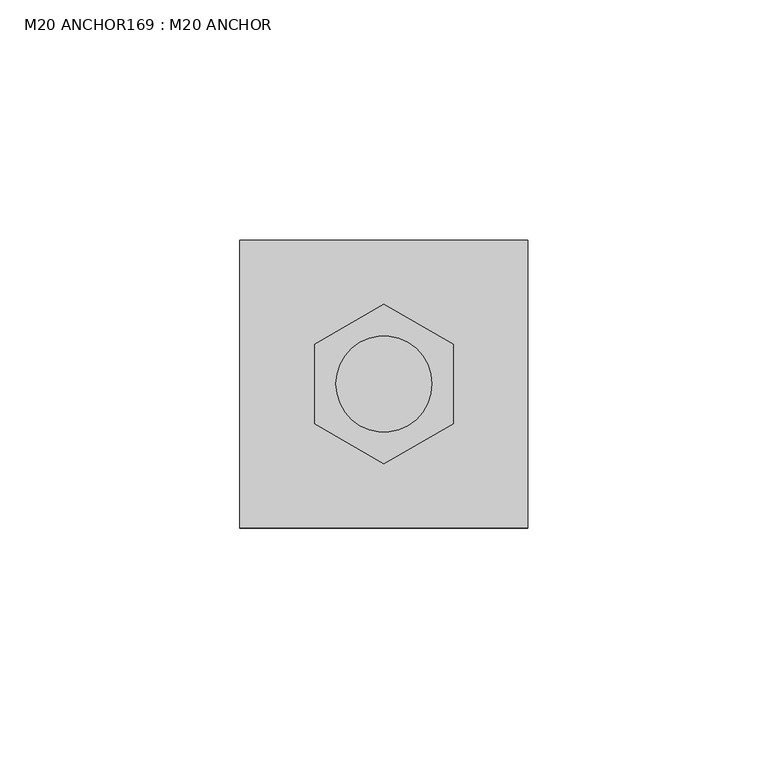
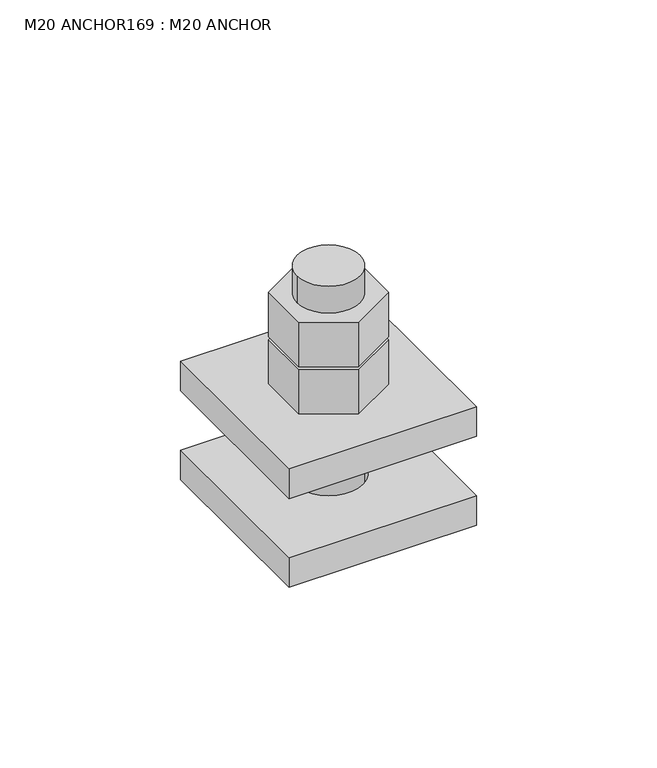
"""IFC4 building model written with IfcOpenShell, lengths in millimetres: fastener geometry, M20 ANCHOR169 : M20 ANCHOR."""

from ifc_helpers import new_model, si_unit, point, frame, frame_2d, origin, place, context, project, spatial, polyline, circle_curve, trimmed, segment, composite_curve, outline, extrude, source, transform, mapped, element, save


def m20_anchor169_m20_anchor_698bed8f(model_context):
    return source(origin(), model_context, "Body", "SweptSolid", [
        extrude(outline(polyline([(6008.0855968, 25545.0952779), (6022.4937158, 25553.4138093), (6036.9018348, 25545.0952779), (6036.9018348, 25528.4582151), (6022.4937158, 25520.1396837), (6008.0855968, 25528.4582151), (6008.0855968, 25545.0952779)]), holes=[composite_curve([segment(trimmed(circle_curve(frame_2d((6022.4937158, 25536.7767465)), 10.0), [point((6032.4937158, 25536.7767465))], [point((6012.4937158, 25536.7767465))], True, "CARTESIAN"), True, "CONTINUOUS"), segment(trimmed(circle_curve(frame_2d((6022.4937158, 25536.7767465)), 10.0), [point((6012.4937158, 25536.7767465))], [point((6032.4937158, 25536.7767465))], True, "CARTESIAN"), True, "CONTINUOUS")], self_intersect=False)]), frame((0.0, 0.0, 246.0), z_axis=(0.0, 0.0, 1.0), x_axis=(1.0, 0.0, 0.0)), (0.0, 0.0, 1.0), 15.0),
        extrude(outline(polyline([(6008.0855968, 25545.0952779), (6022.4937158, 25553.4138093), (6036.9018348, 25545.0952779), (6036.9018348, 25528.4582151), (6022.4937158, 25520.1396837), (6008.0855968, 25528.4582151), (6008.0855968, 25545.0952779)]), holes=[composite_curve([segment(trimmed(circle_curve(frame_2d((6022.4937158, 25536.7767465)), 10.0), [point((6032.4937158, 25536.7767465))], [point((6012.4937158, 25536.7767465))], True, "CARTESIAN"), True, "CONTINUOUS"), segment(trimmed(circle_curve(frame_2d((6022.4937158, 25536.7767465)), 10.0), [point((6012.4937158, 25536.7767465))], [point((6032.4937158, 25536.7767465))], True, "CARTESIAN"), True, "CONTINUOUS")], self_intersect=False)]), frame((0.0, 0.0, 230.0), z_axis=(0.0, 0.0, 1.0), x_axis=(1.0, 0.0, 0.0)), (0.0, 0.0, 1.0), 15.0),
        extrude(outline(composite_curve([segment(trimmed(circle_curve(frame_2d((6022.4937158, 25536.7767465)), 10.0), [point((6032.4937158, 25536.7767465))], [point((6012.4937158, 25536.7767465))], False, "CARTESIAN"), True, "CONTINUOUS"), segment(trimmed(circle_curve(frame_2d((6022.4937158, 25536.7767465)), 10.0), [point((6012.4937158, 25536.7767465))], [point((6032.4937158, 25536.7767465))], False, "CARTESIAN"), True, "CONTINUOUS")], self_intersect=False)), frame((0.0, 0.0, 190.0), z_axis=(0.0, 0.0, 1.0), x_axis=(1.0, 0.0, 0.0)), (0.0, 0.0, 1.0), 80.0),
        extrude(outline(polyline([(5992.4937158, 25566.7767465), (6052.4937158, 25566.7767465), (6052.4937158, 25506.7767465), (5992.4937158, 25506.7767465), (5992.4937158, 25566.7767465)]), holes=[composite_curve([segment(trimmed(circle_curve(frame_2d((6022.4937158, 25536.7767465)), 11.0), [point((6033.4937158, 25536.7767465))], [point((6011.4937158, 25536.7767465))], True, "CARTESIAN"), True, "CONTINUOUS"), segment(trimmed(circle_curve(frame_2d((6022.4937158, 25536.7767465)), 11.0), [point((6011.4937158, 25536.7767465))], [point((6033.4937158, 25536.7767465))], True, "CARTESIAN"), True, "CONTINUOUS")], self_intersect=False)]), frame((0.0, 0.0, 190.0), z_axis=(0.0, 0.0, 1.0), x_axis=(1.0, 0.0, 0.0)), (0.0, 0.0, 1.0), 10.0),
        extrude(outline(polyline([(5992.4937158, 25566.7767465), (6052.4937158, 25566.7767465), (6052.4937158, 25506.7767465), (5992.4937158, 25506.7767465), (5992.4937158, 25566.7767465)]), holes=[composite_curve([segment(trimmed(circle_curve(frame_2d((6022.4937158, 25536.7767465)), 11.0), [point((6033.4937158, 25536.7767465))], [point((6011.4937158, 25536.7767465))], True, "CARTESIAN"), True, "CONTINUOUS"), segment(trimmed(circle_curve(frame_2d((6022.4937158, 25536.7767465)), 11.0), [point((6011.4937158, 25536.7767465))], [point((6033.4937158, 25536.7767465))], True, "CARTESIAN"), True, "CONTINUOUS")], self_intersect=False)]), frame((0.0, 0.0, 220.0), z_axis=(0.0, 0.0, 1.0), x_axis=(1.0, 0.0, 0.0)), (0.0, 0.0, 1.0), 10.0),
    ])


if __name__ == "__main__":
    model = new_model("IFC4")
    model_context = context("Model", 3, world=origin())
    ifc_project = project(units=[si_unit("LENGTHUNIT", "METRE", prefix="MILLI")], contexts=[model_context])
    site = spatial("IfcSite", under=ifc_project)
    building = spatial("IfcBuilding", under=site)
    placement = place(None, origin())
    m20_anchor169_m20_anchor_shape = m20_anchor169_m20_anchor_698bed8f(model_context)
    element("IfcFastener", 1, ObjectType="M20 ANCHOR169 : M20 ANCHOR", at=placement, inside=building, context=model_context, shape_type="MappedRepresentation", body=[
        mapped(m20_anchor169_m20_anchor_shape, transform((0.0, 0.0, 0.0), x_axis=(1.0, 0.0, 0.0), y_axis=(0.0, 1.0, 0.0), z_axis=(0.0, 0.0, 1.0))),
    ])
    save(model, "model.ifc")
